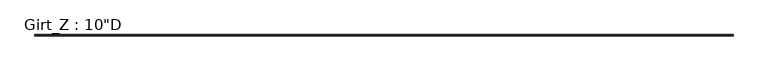
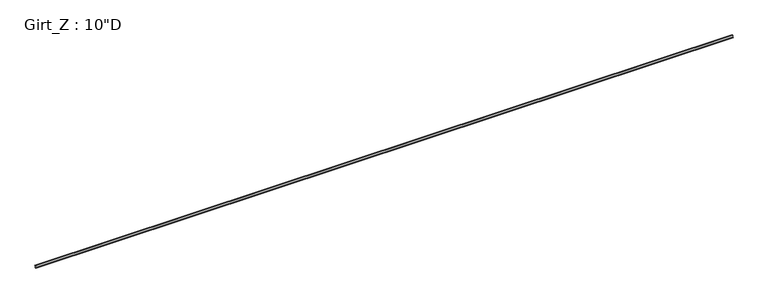
"""IFC4 building model written with IfcOpenShell, lengths in millimetres: beam geometry."""

from ifc_helpers import new_model, si_unit, point, frame, frame_2d, origin, place, context, project, spatial, polyline, circle_curve, trimmed, segment, composite_curve, outline, extrude, source, transform, mapped, element, save


def beam_e6cd5542(model_context):
    return source(origin(), model_context, "Body", "SweptSolid", [
        extrude(outline(composite_curve([segment(polyline([(77.9859375, 127.0), (90.2310415, 112.4068534), (88.1028742, 110.621109), (76.6904765, 124.221875), (3.3005807, 124.221875)]), True, "CONTINUOUS"), segment(trimmed(circle_curve(frame_2d((3.3741066, 122.2381931)), 1.9850441), [point((3.3005807, 124.221875))], [point((1.3890625, 122.2381931))], True, "CARTESIAN"), True, "CONTINUOUS"), segment(polyline([(1.3890625, 122.2381931), (1.3890625, -127.0), (-84.3359375, -127.0), (-96.5810415, -112.4068534), (-94.4528742, -110.621109), (-83.0404765, -124.221875), (-3.2694106, -124.221875)]), True, "CONTINUOUS"), segment(trimmed(circle_curve(frame_2d((-3.3748024, -122.2389339)), 1.9857399), [point((-3.2694106, -124.221875))], [point((-1.3890625, -122.2389339))], True, "CARTESIAN"), True, "CONTINUOUS"), segment(polyline([(-1.3890625, -122.2389339), (-1.3890625, 122.2375)]), True, "CONTINUOUS"), segment(trimmed(circle_curve(frame_2d((3.3734375, 122.2375)), 4.7625), [point((-1.3890625, 122.2375))], [point((3.3734375, 127.0))], False, "CARTESIAN"), True, "CONTINUOUS"), segment(polyline([(3.3734375, 127.0), (77.9859375, 127.0)]), True, "CONTINUOUS")], self_intersect=False)), frame((-44224.90633, 0.0, 0.0), z_axis=(1.0, 0.0, 0.0), x_axis=(0.0, 1.0, 0.0)), (0.0, 0.0, 1.0), 88449.8126599),
    ])


if __name__ == "__main__":
    model = new_model("IFC4")
    model_context = context("Model", 3, world=origin())
    ifc_project = project(units=[si_unit("LENGTHUNIT", "METRE", prefix="MILLI")], contexts=[model_context])
    site = spatial("IfcSite", under=ifc_project)
    building = spatial("IfcBuilding", under=site)
    placement = place(None, origin())
    beam_shape = beam_e6cd5542(model_context)
    element("IfcBeam", 1, ObjectType="Girt_Z : 10\"D", at=placement, inside=building, context=model_context, shape_type="MappedRepresentation", body=[
        mapped(beam_shape, transform((0.0, 0.0, 0.0), x_axis=(1.0, 0.0, 0.0), y_axis=(0.0, 1.0, 0.0), z_axis=(0.0, 0.0, 1.0))),
    ])
    save(model, "model.ifc")

# Revit data of these elements
# Type "Girt_Z : 10\"D"
#   half leg = 0' - 1 11/16"
#   Web_Thickness = 0' - 0 7/64"
#   Length [instance default] = 10' - 0"
#   Leg_2 = 0' - 3 3/8"
#   Leg_1 = 0' - 3 1/8"
#   Height = 0' - 10"
#   Structural Material [instance default] = none
# Element 1 (IfcBeam, "Girt_Z : 10\"D")
#   Structural Material = STRUCTURAL STEEL - SEE STRUCT. DWGS
#   Materials on its faces: "STRUCTURAL STEEL - SEE STRUCT. DWGS"
# Materials
#   "STRUCTURAL STEEL - SEE STRUCT. DWGS": class "Metal", colour RGB 137 146 153, transparency 0, Description = "Steel, mill finish", Cost = 0
